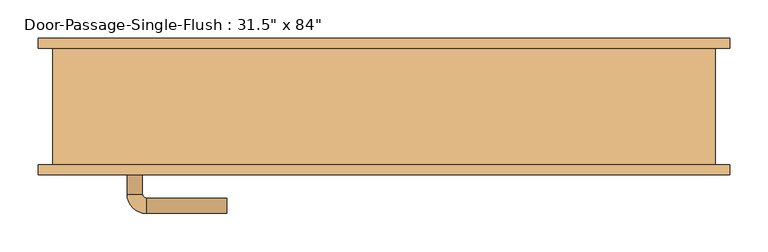
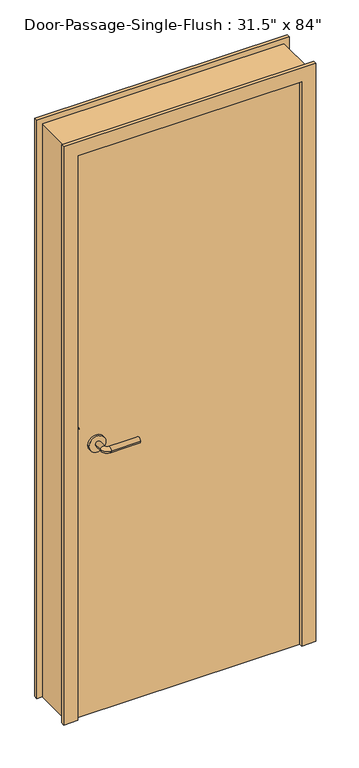
"""IFC4 building model written with IfcOpenShell, lengths in millimetres: door geometry."""

from ifc_helpers import new_model, si_unit, point, frame, frame_2d, origin, origin_with_axes, place, context, project, spatial, polyline, circle_curve, ellipse_curve, trimmed, segment, composite_curve, outline, extrude, faceted_brep, source, transform, mapped, element, save
from ifc_brep_helpers import plane_surface, cylinder_surface, revolved_surface, advanced_brep


def door_b02f4eba(model_context):
    return source(origin(), model_context, "Body", "SolidModel", [
        advanced_brep(
        [(-335.040625, -23.75, 1016.0), (-315.040625, -23.75, 1016.0), (-335.040625, 6.25, 1016.0), (-315.040625, 6.25, 1016.0), (-310.040625, 11.25, 1016.0), (-310.040625, 31.25, 1016.0), (-205.040625, 31.25, 1016.0), (-205.040625, 11.25, 1016.0)],
        [
            (0, 1, circle_curve(frame((-325.040625, -23.75, 1016.0), z_axis=(0.0, -1.0, 0.0), x_axis=(1.0, 0.0, 0.0)), 10.0)),
            (1, 0, circle_curve(frame((-325.040625, -23.75, 1016.0), z_axis=(0.0, -1.0, 0.0), x_axis=(1.0, 0.0, 0.0)), 10.0)),
            (0, 2),
            (2, 3, circle_curve(frame((-325.040625, 6.25, 1016.0), z_axis=(0.0, -1.0, 0.0), x_axis=(1.0, 0.0, 0.0)), 10.0)),
            (3, 1),
            (3, 2, circle_curve(frame((-325.040625, 6.25, 1016.0), z_axis=(0.0, -1.0, 0.0), x_axis=(1.0, 0.0, 0.0)), 10.0)),
            (4, 3, circle_curve(frame((-310.040625, 6.25, 1016.0), z_axis=(0.0, 0.0, 1.0), x_axis=(-1.0, 0.0, 0.0)), 5.0)),
            (2, 5, circle_curve(frame((-310.040625, 6.25, 1016.0), z_axis=(0.0, 0.0, -1.0), x_axis=(-1.0, 0.0, 0.0)), 25.0)),
            (5, 4, circle_curve(frame((-310.040625, 21.25, 1016.0), z_axis=(-1.0, 0.0, 0.0), x_axis=(0.0, -1.0, 0.0)), 10.0)),
            (4, 5, circle_curve(frame((-310.040625, 21.25, 1016.0), z_axis=(-1.0, 0.0, 0.0), x_axis=(0.0, -1.0, 0.0)), 10.0)),
            (6, 7, circle_curve(frame((-205.040625, 21.25, 1016.0), z_axis=(1.0, 0.0, 0.0), x_axis=(0.0, -1.0, 0.0)), 10.0)),
            (7, 6, circle_curve(frame((-205.040625, 21.25, 1016.0), z_axis=(1.0, 0.0, 0.0), x_axis=(0.0, -1.0, 0.0)), 10.0)),
            (5, 6),
            (7, 4),
        ],
        [
            plane_surface(frame((-325.040625, -23.75, 1016.0), z_axis=(0.0, -1.0, 0.0), x_axis=(0.0, 0.0, 1.0))),
            cylinder_surface(frame((-325.040625, -23.75, 1016.0), z_axis=(0.0, -1.0, 0.0), x_axis=(1.0, 0.0, 0.0)), 10.0),
            revolved_surface(trimmed(ellipse_curve(frame((-325.040625, 6.25, 1016.0), z_axis=(0.0, -1.0, 0.0), x_axis=(1.0, 0.0, 0.0)), 10.0, 10.0), [point((-335.040625, 6.25, 1016.0))], [point((-315.040625, 6.25, 1016.0))], True, "CARTESIAN"), (-310.040625, 6.25, 1016.0), (0.0, 0.0, -1.0)),
            revolved_surface(trimmed(ellipse_curve(frame((-325.040625, 6.25, 1016.0), z_axis=(0.0, -1.0, 0.0), x_axis=(1.0, 0.0, 0.0)), 10.0, 10.0), [point((-315.040625, 6.25, 1016.0))], [point((-335.040625, 6.25, 1016.0))], True, "CARTESIAN"), (-310.040625, 6.25, 1016.0), (0.0, 0.0, -1.0)),
            plane_surface(frame((-205.040625, 21.25, 1016.0), z_axis=(1.0, 0.0, 0.0), x_axis=(0.0, 0.0, 1.0))),
            cylinder_surface(frame((-310.040625, 21.25, 1016.0), z_axis=(-1.0, 0.0, 0.0), x_axis=(0.0, -1.0, 0.0)), 10.0),
        ],
        [
            (0, [[1, 2]]),
            (1, [[-1, 3, 4, 5]]),
            (1, [[-2, -5, 6, -3]]),
            (2, [[7, -4, 8, 9]]),
            (3, [[-8, -6, -7, 10]]),
            (4, [[11, 12]]),
            (5, [[-9, 13, -12, 14]]),
            (5, [[-10, -14, -11, -13]]),
        ],
    ),
        extrude(outline(composite_curve([segment(trimmed(circle_curve(frame_2d((1016.0, -327.540625)), 30.0), [point((1016.0, -357.540625))], [point((1016.0, -297.540625))], False, "CARTESIAN"), True, "CONTINUOUS"), segment(trimmed(circle_curve(frame_2d((1016.0, -327.540625)), 30.0), [point((1016.0, -297.540625))], [point((1016.0, -357.540625))], False, "CARTESIAN"), True, "CONTINUOUS")], self_intersect=False)), frame((0.0, -31.75, 0.0), z_axis=(0.0, 1.0, 0.0), x_axis=(0.0, 0.0, 1.0)), (0.0, 0.0, 1.0), 8.0),
        advanced_brep(
        [(-335.040625, -90.55, 1016.0), (-315.040625, -90.55, 1016.0), (-315.040625, -120.55, 1016.0), (-335.040625, -120.55, 1016.0), (-310.040625, -125.55, 1016.0), (-310.040625, -145.55, 1016.0), (-205.040625, -145.55, 1016.0), (-205.040625, -125.55, 1016.0)],
        [
            (0, 1, circle_curve(frame((-325.040625, -90.55, 1016.0), z_axis=(0.0, 1.0, 0.0), x_axis=(1.0, 0.0, 0.0)), 10.0)),
            (1, 0, circle_curve(frame((-325.040625, -90.55, 1016.0), z_axis=(0.0, 1.0, 0.0), x_axis=(1.0, 0.0, 0.0)), 10.0)),
            (1, 2),
            (2, 3, circle_curve(frame((-325.040625, -120.55, 1016.0), z_axis=(0.0, 1.0, 0.0), x_axis=(1.0, 0.0, 0.0)), 10.0)),
            (3, 0),
            (3, 2, circle_curve(frame((-325.040625, -120.55, 1016.0), z_axis=(0.0, 1.0, 0.0), x_axis=(1.0, 0.0, 0.0)), 10.0)),
            (4, 5, circle_curve(frame((-310.040625, -135.55, 1016.0), z_axis=(-1.0, 0.0, 0.0), x_axis=(0.0, 1.0, 0.0)), 10.0)),
            (5, 3, circle_curve(frame((-310.040625, -120.55, 1016.0), z_axis=(0.0, 0.0, -1.0), x_axis=(-1.0, 0.0, 0.0)), 25.0)),
            (2, 4, circle_curve(frame((-310.040625, -120.55, 1016.0), z_axis=(0.0, 0.0, 1.0), x_axis=(-1.0, 0.0, 0.0)), 5.0)),
            (5, 4, circle_curve(frame((-310.040625, -135.55, 1016.0), z_axis=(-1.0, 0.0, 0.0), x_axis=(0.0, 1.0, 0.0)), 10.0)),
            (6, 7, circle_curve(frame((-205.040625, -135.55, 1016.0), z_axis=(1.0, 0.0, 0.0), x_axis=(0.0, 1.0, 0.0)), 10.0)),
            (7, 6, circle_curve(frame((-205.040625, -135.55, 1016.0), z_axis=(1.0, 0.0, 0.0), x_axis=(0.0, 1.0, 0.0)), 10.0)),
            (4, 7),
            (6, 5),
        ],
        [
            plane_surface(frame((-325.040625, -90.55, 1016.0), z_axis=(0.0, 1.0, 0.0), x_axis=(0.0, 0.0, 1.0))),
            cylinder_surface(frame((-325.040625, -90.55, 1016.0), z_axis=(0.0, 1.0, 0.0), x_axis=(1.0, 0.0, 0.0)), 10.0),
            revolved_surface(trimmed(ellipse_curve(frame((-325.040625, -120.55, 1016.0), z_axis=(0.0, -1.0, 0.0), x_axis=(1.0, 0.0, 0.0)), 10.0, 10.0), [point((-335.040625, -120.55, 1016.0))], [point((-315.040625, -120.55, 1016.0))], True, "CARTESIAN"), (-310.040625, -120.55, 1016.0), (0.0, 0.0, -1.0)),
            revolved_surface(trimmed(ellipse_curve(frame((-325.040625, -120.55, 1016.0), z_axis=(0.0, -1.0, 0.0), x_axis=(1.0, 0.0, 0.0)), 10.0, 10.0), [point((-315.040625, -120.55, 1016.0))], [point((-335.040625, -120.55, 1016.0))], True, "CARTESIAN"), (-310.040625, -120.55, 1016.0), (0.0, 0.0, -1.0)),
            plane_surface(frame((-205.040625, -135.55, 1016.0), z_axis=(1.0, 0.0, 0.0), x_axis=(0.0, 0.0, 1.0))),
            cylinder_surface(frame((-310.040625, -135.55, 1016.0), z_axis=(-1.0, 0.0, 0.0), x_axis=(0.0, 1.0, 0.0)), 10.0),
        ],
        [
            (0, [[1, 2]]),
            (1, [[3, 4, 5, -2]]),
            (1, [[-5, 6, -3, -1]]),
            (2, [[7, 8, -4, 9]]),
            (3, [[10, -9, -6, -8]]),
            (4, [[11, 12]]),
            (5, [[13, -11, 14, -7]]),
            (5, [[-14, -12, -13, -10]]),
        ],
    ),
        extrude(outline(composite_curve([segment(trimmed(circle_curve(frame_2d((1016.0, -327.540625)), 30.0), [point((1016.0, -357.540625))], [point((1016.0, -297.540625))], False, "CARTESIAN"), True, "CONTINUOUS"), segment(trimmed(circle_curve(frame_2d((1016.0, -327.540625)), 30.0), [point((1016.0, -297.540625))], [point((1016.0, -357.540625))], False, "CARTESIAN"), True, "CONTINUOUS")], self_intersect=False)), frame((0.0, -90.55, 0.0), z_axis=(0.0, 1.0, 0.0), x_axis=(0.0, 0.0, 1.0)), (0.0, 0.0, 1.0), 8.0),
        faceted_brep([(400.05, -95.25, 0.0), (400.05, -26.9875, 0.0), (384.175, -26.9875, 0.0), (384.175, 11.1125, 0.0), (400.05, 11.1125, 0.0), (400.05, 82.55, 0.0), (450.85, 82.55, 0.0), (450.85, 69.85, 0.0), (431.8, 69.85, 0.0), (431.8, -82.55, 0.0), (450.85, -82.55, 0.0), (450.85, -95.25, 0.0), (450.85, -95.25, 2184.4), (-450.85, -95.25, 2184.4), (-450.85, -95.25, 0.0), (-400.05, -95.25, 0.0), (-400.05, -95.25, 2133.6), (400.05, -95.25, 2133.6), (450.85, -82.55, 2184.4), (431.8, -82.55, 2165.35), (-431.8, -82.55, 2165.35), (-431.8, -82.55, 0.0), (-450.85, -82.55, 0.0), (-450.85, -82.55, 2184.4), (431.8, 69.85, 2165.35), (450.85, 69.85, 2184.4), (-450.85, 69.85, 2184.4), (-450.85, 69.85, 0.0), (-431.8, 69.85, 0.0), (-431.8, 69.85, 2165.35), (450.85, 82.55, 2184.4), (400.05, 82.55, 2133.6), (-400.05, 82.55, 2133.6), (-400.05, 82.55, 0.0), (-450.85, 82.55, 0.0), (-450.85, 82.55, 2184.4), (400.05, 11.1125, 2133.6), (384.175, 11.1125, 2117.725), (-384.175, 11.1125, 2117.725), (-384.175, 11.1125, 0.0), (-400.05, 11.1125, 0.0), (-400.05, 11.1125, 2133.6), (384.175, -26.9875, 2117.725), (400.05, -26.9875, 2133.6), (-400.05, -26.9875, 2133.6), (-400.05, -26.9875, 0.0), (-384.175, -26.9875, 0.0), (-384.175, -26.9875, 2117.725)], [[[0, 1, 2, 3, 4, 5, 6, 7, 8, 9, 10, 11]], [[11, 12, 13, 14, 15, 16, 17, 0]], [[10, 18, 12, 11]], [[9, 19, 20, 21, 22, 23, 18, 10]], [[8, 24, 19, 9]], [[7, 25, 26, 27, 28, 29, 24, 8]], [[6, 30, 25, 7]], [[5, 31, 32, 33, 34, 35, 30, 6]], [[4, 36, 31, 5]], [[3, 37, 38, 39, 40, 41, 36, 4]], [[2, 42, 37, 3]], [[1, 43, 44, 45, 46, 47, 42, 2]], [[0, 17, 43, 1]], [[18, 23, 13, 12]], [[24, 29, 20, 19]], [[30, 35, 26, 25]], [[36, 41, 32, 31]], [[42, 47, 38, 37]], [[17, 16, 44, 43]], [[15, 14, 22, 21, 28, 27, 34, 33, 40, 39, 46, 45]], [[23, 22, 14, 13]], [[29, 28, 21, 20]], [[35, 34, 27, 26]], [[41, 40, 33, 32]], [[47, 46, 39, 38]], [[16, 15, 45, 44]]]),
        extrude(outline(polyline([(400.05, -31.75), (400.05, -82.55), (-400.05, -82.55), (-400.05, -31.75), (400.05, -31.75)])), origin_with_axes(), (0.0, 0.0, 1.0), 2133.6),
    ])


if __name__ == "__main__":
    model = new_model("IFC4")
    model_context = context("Model", 3, world=origin())
    ifc_project = project(units=[si_unit("LENGTHUNIT", "METRE", prefix="MILLI")], contexts=[model_context])
    site = spatial("IfcSite", under=ifc_project)
    building = spatial("IfcBuilding", under=site)
    placement = place(None, origin())
    door_shape = door_b02f4eba(model_context)
    element("IfcDoor", 1, ObjectType="Door-Passage-Single-Flush : 31.5\" x 84\"", at=placement, inside=building, context=model_context, shape_type="MappedRepresentation", body=[
        mapped(door_shape, transform((0.0, 0.0, 0.0), x_axis=(1.0, 0.0, 0.0), y_axis=(0.0, 1.0, 0.0), z_axis=(0.0, 0.0, 1.0))),
    ])
    save(model, "model.ifc")

# Revit data of these elements
# Type "Door-Passage-Single-Flush : 31.5\" x 84\""
#   Type Mark = "24"
#   Assembly Code = "C1020"
#   Analytic Construction = "Wooden"
#   Thickness = 0' - 2"
#   Thermal Resistance (R) = 2.5876 (h·ft²·°F)/BTU
#   Swing Angle [instance default] = 90.00°
#   Strike Height = 3' - 4"
#   Rough Width [instance default] = 2' - 11 1/2"
#   Rough Height [instance default] = 7' - 4"
#   Masonry Inset [instance default] = 0' - 1"
#   Masonry Frame Depth = 0' - 5 3/4"
#   MF Opening Width [instance default] = 0' - 4"
#   MF Opening Height [instance default] = 0' - 4"
#   Inset Calculate [instance default] = 0' - 4"
#   Heat Transfer Coefficient (U) = 0.3865 BTU/(h·ft²·°F)
#   Height = 7' - 0"
#   Width = 2' - 7 1/2"
#   Masonry Frame [instance default] = yes
#   Dry Wall Frame [instance default] = no
#   Panel Material = Wood - Birch
#   Frame Material = Door - Frame
#   Door Handle Material = Aluminum
#   Visual Light Transmittance = 0
#   Solar Heat Gain Coefficient = 0
#   Function = (empty or 0)
#   Wall Closure = (empty or 0)
# Element 1 (IfcDoor, "Door-Passage-Single-Flush : 31.5\" x 84\"")
#   Rough Width = 2' - 10"
#   Rough Height = 7' - 1 1/4"
#   MF Opening Width = 0' - 2 1/2"
#   MF Opening Height = 0' - 1 1/4"
#   Inset Calculate = 0' - 3"
#   Masonry Frame = no
#   Dry Wall Frame = yes
#   Materials on its faces: "Door - Frame", "Aluminum", "Wood - Birch"
# Materials
#   "Wood - Birch": class "Unassigned", colour RGB 224 178 126, transparency 0
#   "Door - Frame": class "Unassigned", colour RGB 118 70 51, transparency 0
#   "Aluminum": class "Metal", colour RGB 244 244 244, transparency 0, Description = "Aluminum 6061", Cost = 0
